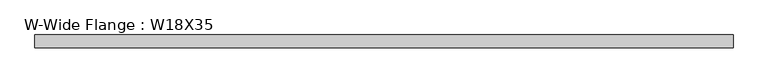
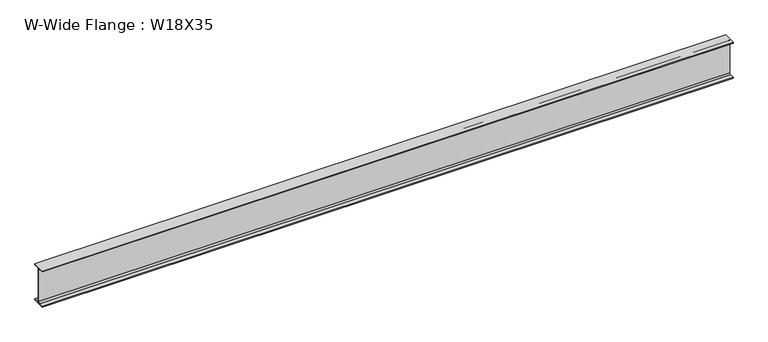
"""IFC4 building model written with IfcOpenShell, lengths in millimetres: beam geometry, W-Wide Flange : W18X35."""

import ifcopenshell
import ifcopenshell.guid

model = None  # the IFC model being written
_history = None  # IfcOwnerHistory: only IFC2X3 demands one
_inside = {}  # id of a spatial element -> (the spatial element, [elements in it])
_under = {}  # id of a project, library or spatial element -> (it, [spatial elements below it])
_declared = {}  # id of a project -> (the project, [libraries it declares])
_typed = {}  # id of a type object -> (the type object, [elements of that type])
_made_of = {}  # id of a material, layer set ... -> (it, [elements and type objects made of it])


def new_model(schema):
    """Start an empty IFC model of exactly this schema.

    Asked for "IFC4X3", IfcOpenShell would pick the latest addendum, in which some entities
    have other attributes; the version numbers below select the first issue.
    IFC2X3 requires an IfcOwnerHistory on every rooted entity: one is made here for all.
    """
    global model, _history
    if schema == "IFC4X3":
        model = ifcopenshell.file(schema_version=(4, 3, 0, 0))
    else:
        model = ifcopenshell.file(schema=schema)
    _inside.clear()
    _under.clear()
    _declared.clear()
    _typed.clear()
    _made_of.clear()
    _history = None
    if model.schema == "IFC2X3":
        org = make("IfcOrganization", Name="unknown")
        user = make(
            "IfcPersonAndOrganization",
            ThePerson=make("IfcPerson", FamilyName="unknown"),
            TheOrganization=org,
        )
        app = make(
            "IfcApplication",
            ApplicationDeveloper=org,
            Version="unknown",
            ApplicationFullName="unknown",
            ApplicationIdentifier="unknown",
        )
        _history = make(
            "IfcOwnerHistory",
            OwningUser=user,
            OwningApplication=app,
            ChangeAction="ADDED",
            CreationDate=0,
        )
    return model


def make(cls, **values):
    """One entity of the class cls with the attributes given. An attribute that is None is left unset."""
    return model.create_entity(
        cls, **{name: value for name, value in values.items() if value is not None}
    )


def rooted(cls, **values):
    """An entity with a GlobalId (a new one), such as an element, a storey or a relation."""
    return make(cls, GlobalId=ifcopenshell.guid.new(), OwnerHistory=_history, **values)


def si_unit(unit_type, name, prefix=None):
    """IfcSIUnit, for example si_unit("LENGTHUNIT", "METRE", prefix="MILLI")."""
    return make("IfcSIUnit", UnitType=unit_type, Prefix=prefix, Name=name)


def assignment(units):
    """IfcUnitAssignment: the units of a project."""
    return None if units is None else make("IfcUnitAssignment", Units=units)


def point(xyz):
    """IfcCartesianPoint."""
    return None if xyz is None else make("IfcCartesianPoint", Coordinates=xyz)


def direction(xyz):
    """IfcDirection."""
    return None if xyz is None else make("IfcDirection", DirectionRatios=xyz)


def frame(location, z_axis=None, x_axis=None):
    """IfcAxis2Placement3D, a coordinate frame: its origin and axes. An axis left out is left unset."""
    return make(
        "IfcAxis2Placement3D",
        Location=point(location),
        Axis=direction(z_axis),
        RefDirection=direction(x_axis),
    )


def frame_2d(location, x_axis=None):
    """IfcAxis2Placement2D, a coordinate frame in the plane: its origin and x axis."""
    return make(
        "IfcAxis2Placement2D", Location=point(location), RefDirection=direction(x_axis)
    )


def origin():
    """The frame at (0, 0, 0) with its axes left unset."""
    return frame((0.0, 0.0, 0.0))


def place(relative_to, where):
    """IfcLocalPlacement: puts the frame where relative to a parent placement (None: the world)."""
    return make(
        "IfcLocalPlacement", PlacementRelTo=relative_to, RelativePlacement=where
    )


def context(
    kind, dimensions, precision=None, world=None, true_north=None, identifier=None
):
    """IfcGeometricRepresentationContext, for example the 3D "Model" context."""
    return make(
        "IfcGeometricRepresentationContext",
        ContextIdentifier=identifier,
        ContextType=kind,
        CoordinateSpaceDimension=dimensions,
        Precision=precision,
        WorldCoordinateSystem=world,
        TrueNorth=true_north,
    )


def project(units=None, contexts=None):
    """IfcProject with its units and contexts."""
    return rooted(
        "IfcProject",
        Name="project",
        RepresentationContexts=contexts,
        UnitsInContext=assignment(units),
    )


def spatial(cls, under=None, at=None, **own):
    """A site, building, storey or space (cls), placed at a placement, below another one or the project."""
    s = rooted(cls, ObjectPlacement=at, **own)
    if under is not None:
        _under.setdefault(under.id(), (under, []))[1].append(s)
    return s


def polyline(points):
    """IfcPolyline through the points."""
    return make("IfcPolyline", Points=[point(p) for p in points])


def circle_curve(where, radius):
    """IfcCircle in the frame where."""
    return make("IfcCircle", Position=where, Radius=radius)


def trimmed(basis, trim1, trim2, sense, master):
    """IfcTrimmedCurve: the piece of a basis curve between two trims."""
    return make(
        "IfcTrimmedCurve",
        BasisCurve=basis,
        Trim1=trim1,
        Trim2=trim2,
        SenseAgreement=sense,
        MasterRepresentation=master,
    )


def segment(curve, same_sense, transition):
    """IfcCompositeCurveSegment."""
    return make(
        "IfcCompositeCurveSegment",
        Transition=transition,
        SameSense=same_sense,
        ParentCurve=curve,
    )


def composite_curve(segments, self_intersect=None):
    """IfcCompositeCurve: segments joined end to end."""
    return make("IfcCompositeCurve", Segments=segments, SelfIntersect=self_intersect)


def outline(outer, holes=None, kind="AREA"):
    """IfcArbitraryClosedProfileDef: a profile drawn as a closed curve; with holes, ...WithVoids."""
    if holes is None:
        return make("IfcArbitraryClosedProfileDef", ProfileType=kind, OuterCurve=outer)
    return make(
        "IfcArbitraryProfileDefWithVoids",
        ProfileType=kind,
        OuterCurve=outer,
        InnerCurves=holes,
    )


def extrude(swept, where, along, depth):
    """IfcExtrudedAreaSolid: the profile swept, set in the frame where, extruded along a direction by depth."""
    return make(
        "IfcExtrudedAreaSolid",
        SweptArea=swept,
        Position=where,
        ExtrudedDirection=direction(along),
        Depth=depth,
    )


def shape(context_of_items, identifier, shape_type, items):
    """IfcShapeRepresentation: the items that make up one representation, for example the "Body"."""
    return make(
        "IfcShapeRepresentation",
        ContextOfItems=context_of_items,
        RepresentationIdentifier=identifier,
        RepresentationType=shape_type,
        Items=items,
    )


def source(mapping_origin, context_of_items, identifier, shape_type, items):
    """IfcRepresentationMap: a shape defined once, which mapped items show again and again."""
    return make(
        "IfcRepresentationMap",
        MappingOrigin=mapping_origin,
        MappedRepresentation=shape(context_of_items, identifier, shape_type, items),
    )


def transform(
    local_origin,
    x_axis=None,
    y_axis=None,
    z_axis=None,
    scale=None,
    scale2=None,
    scale3=None,
    uniform=True,
):
    """IfcCartesianTransformationOperator3D, or its non-uniform kind. x_axis, y_axis, z_axis: its Axis1, 2, 3."""
    if uniform:
        return make(
            "IfcCartesianTransformationOperator3D",
            Axis1=direction(x_axis),
            Axis2=direction(y_axis),
            LocalOrigin=point(local_origin),
            Scale=scale,
            Axis3=direction(z_axis),
        )
    return make(
        "IfcCartesianTransformationOperator3DnonUniform",
        Axis1=direction(x_axis),
        Axis2=direction(y_axis),
        LocalOrigin=point(local_origin),
        Scale=scale,
        Axis3=direction(z_axis),
        Scale2=scale2,
        Scale3=scale3,
    )


def mapped(mapping_source, mapping_target):
    """IfcMappedItem: shows the shape of a source again, moved by a transform."""
    return make(
        "IfcMappedItem", MappingSource=mapping_source, MappingTarget=mapping_target
    )


def made_of(thing, what):
    """Note that an element or type object is made of a material, layer set ...; save() writes the relation."""
    if what is not None:
        _made_of.setdefault(what.id(), (what, []))[1].append(thing)
    return thing


def element(
    cls,
    number,
    at=None,
    inside=None,
    cuts=None,
    type_object=None,
    material=None,
    context=None,
    identifier="Body",
    shape_type=None,
    held_by="IfcProductDefinitionShape",
    body=None,
    shapes=None,
    **own,
):
    """One element of the class cls, such as IfcWall. Its Tag is "e" and its number.

    at: its placement. inside: the storey or other place that contains it. cuts: it is an
    opening in that element (IfcRelVoidsElement). A single representation is given by context,
    identifier, shape_type and body (its items); several are given by shapes. held_by: the class
    of the entity that holds the representations. save() writes the other relations.
    """
    e = rooted(cls, Tag="e%d" % number, ObjectPlacement=at, **own)
    if body is not None:
        shapes = [shape(context, identifier, shape_type, body)]
    if shapes is not None:
        e.Representation = make(held_by, Representations=shapes)
    if inside is not None:
        _inside.setdefault(inside.id(), (inside, []))[1].append(e)
    if cuts is not None:
        rooted(
            "IfcRelVoidsElement", RelatingBuildingElement=cuts, RelatedOpeningElement=e
        )
    if type_object is not None:
        _typed.setdefault(type_object.id(), (type_object, []))[1].append(e)
    return made_of(e, material)


def aggregate(whole, parts):
    """IfcRelAggregates: a whole, such as a stair, and the parts it consists of."""
    return rooted("IfcRelAggregates", RelatingObject=whole, RelatedObjects=parts)


def save(model, path):
    """Write the relations noted so far, then the file.

    IfcRelAggregates (storeys below a building ...), IfcRelContainedInSpatialStructure (elements
    in a storey), IfcRelDefinesByType, IfcRelAssociatesMaterial and IfcRelDeclares: one each for
    every whole, place, type object, material and project.
    """
    for whole, parts in _under.values():
        aggregate(whole, parts)
    for where, things in _inside.values():
        rooted(
            "IfcRelContainedInSpatialStructure",
            RelatedElements=things,
            RelatingStructure=where,
        )
    for kind, things in _typed.values():
        rooted("IfcRelDefinesByType", RelatedObjects=things, RelatingType=kind)
    for what, things in _made_of.values():
        rooted("IfcRelAssociatesMaterial", RelatedObjects=things, RelatingMaterial=what)
    for by, libraries in _declared.values():
        rooted("IfcRelDeclares", RelatingContext=by, RelatedDefinitions=libraries)
    model.write(path)


def w_wide_flange_w18x35_2abc70fe(model_context):
    return source(origin(), model_context, "Body", "SweptSolid", [
        extrude(outline(composite_curve([segment(polyline([(76.2, -213.995), (76.2, -224.79), (-76.2, -224.79), (-76.2, -213.995), (-21.59, -213.995)]), True, "CONTINUOUS"), segment(trimmed(circle_curve(frame_2d((-21.59, -196.215)), 17.78), [point((-21.59, -213.995))], [point((-3.81, -196.215))], True, "CARTESIAN"), True, "CONTINUOUS"), segment(polyline([(-3.81, -196.215), (-3.81, 196.215)]), True, "CONTINUOUS"), segment(trimmed(circle_curve(frame_2d((-21.59, 196.215)), 17.78), [point((-3.81, 196.215))], [point((-21.59, 213.995))], True, "CARTESIAN"), True, "CONTINUOUS"), segment(polyline([(-21.59, 213.995), (-76.2, 213.995), (-76.2, 224.79), (76.2, 224.79), (76.2, 213.995), (21.59, 213.995)]), True, "CONTINUOUS"), segment(trimmed(circle_curve(frame_2d((21.59, 196.215)), 17.78), [point((21.59, 213.995))], [point((3.81, 196.215))], True, "CARTESIAN"), True, "CONTINUOUS"), segment(polyline([(3.81, 196.215), (3.81, -196.215)]), True, "CONTINUOUS"), segment(trimmed(circle_curve(frame_2d((21.59, -196.215)), 17.78), [point((3.81, -196.215))], [point((21.59, -213.995))], True, "CARTESIAN"), True, "CONTINUOUS"), segment(polyline([(21.59, -213.995), (76.2, -213.995)]), True, "CONTINUOUS")], self_intersect=False)), frame((-4076.7, 0.0, 0.0), z_axis=(1.0, 0.0, 0.0), x_axis=(0.0, 1.0, 0.0)), (0.0, 0.0, 1.0), 8153.4),
    ])


if __name__ == "__main__":
    model = new_model("IFC4")
    model_context = context("Model", 3, world=origin())
    ifc_project = project(units=[si_unit("LENGTHUNIT", "METRE", prefix="MILLI")], contexts=[model_context])
    site = spatial("IfcSite", under=ifc_project)
    building = spatial("IfcBuilding", under=site)
    placement = place(None, origin())
    w_wide_flange_w18x35_shape = w_wide_flange_w18x35_2abc70fe(model_context)
    element("IfcBeam", 1, ObjectType="W-Wide Flange : W18X35", at=placement, inside=building, context=model_context, shape_type="MappedRepresentation", body=[
        mapped(w_wide_flange_w18x35_shape, transform((0.0, 0.0, 0.0), x_axis=(1.0, 0.0, 0.0), y_axis=(0.0, 1.0, 0.0), z_axis=(0.0, 0.0, 1.0))),
    ])
    save(model, "model.ifc")

# Revit data of these elements
# Type "W-Wide Flange : W18X35"
#   Assembly Code = "B10"
#   W = 35
#   Length [instance default] = 5' - 0"
#   bf = 0' - 6"
#   d = 1' - 5.7"
#   k = 0' - 1 1/8"
#   k2 = 0' - 0.7"
#   tf = 0' - 0.425"
#   tw = 0' - 0.3"
#   A = 0.0715278 SF
#   Structural Material [instance default] = Steel ASTM A992
# Element 1 (IfcBeam, "W-Wide Flange : W18X35")
#   Materials on its faces: "Steel ASTM A992"
# Materials
#   "Steel ASTM A992": class "Metal", colour RGB 199 199 199, transparency 0, Description = "Structural steel 50ksi", Cost = 0
